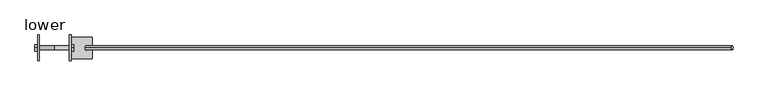
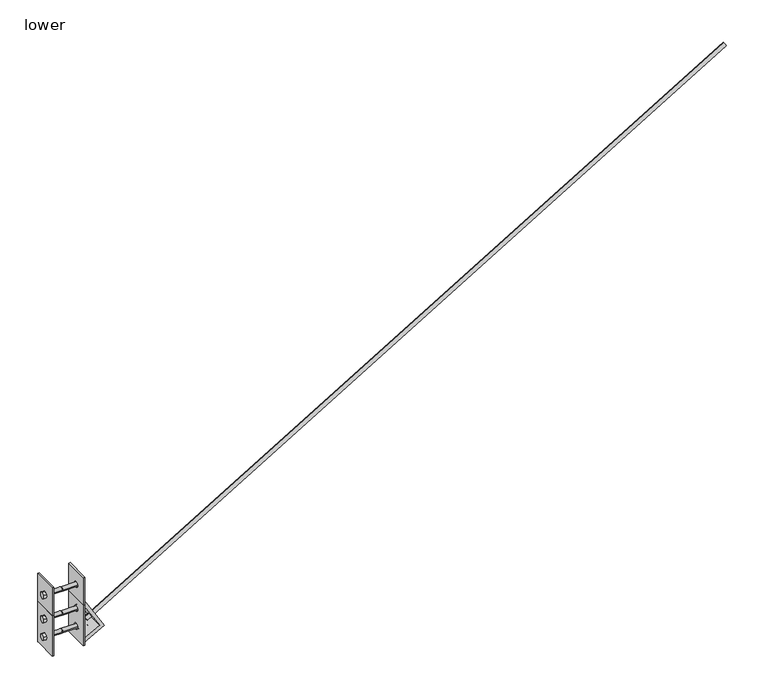
"""IFC4 building model written with IfcOpenShell, lengths in millimetres: fastener geometry, 060523 - W_P_C - Fastenings - Column Base & Top with X Bracing - Custom : lower."""

from ifc_helpers import new_model, si_unit, point, frame, frame_2d, origin, place, context, project, spatial, polyline, circle_curve, trimmed, segment, composite_curve, outline, extrude, source, transform, mapped, element, save
from ifc_brep_helpers import plane_surface, revolved_surface, advanced_brep


def lower_b6991e01(model_context):
    return source(origin(), model_context, "Body", "SolidModel", [
        extrude(outline(polyline([(-14.2875, 168.586392), (0.0, 176.8352839), (14.2875, 168.586392), (14.2875, 152.088608), (0.0, 143.8397161), (-14.2875, 152.088608), (-14.2875, 168.586392)])), frame((-90.4875, 0.0, 0.0), z_axis=(1.0, 0.0, 0.0), x_axis=(0.0, 1.0, 0.0)), (0.0, 0.0, 1.0), 12.7),
        extrude(outline(composite_curve([segment(trimmed(circle_curve(frame_2d((0.0, 160.3375)), 9.525), [point((-9.525, 160.3375))], [point((9.525, 160.3375))], False, "CARTESIAN"), True, "CONTINUOUS"), segment(trimmed(circle_curve(frame_2d((0.0, 160.3375)), 9.525), [point((9.525, 160.3375))], [point((-9.525, 160.3375))], False, "CARTESIAN"), True, "CONTINUOUS")], self_intersect=False)), frame((-77.7875, 0.0, 0.0), z_axis=(1.0, 0.0, 0.0), x_axis=(0.0, 1.0, 0.0)), (0.0, 0.0, 1.0), 76.2),
        extrude(outline(polyline([(-14.2875, 79.686392), (0.0, 87.9352839), (14.2875, 79.686392), (14.2875, 63.188608), (0.0, 54.9397161), (-14.2875, 63.188608), (-14.2875, 79.686392)])), frame((-90.4875, 0.0, 0.0), z_axis=(1.0, 0.0, 0.0), x_axis=(0.0, 1.0, 0.0)), (0.0, 0.0, 1.0), 12.7),
        extrude(outline(composite_curve([segment(trimmed(circle_curve(frame_2d((0.0, 71.4375)), 9.525), [point((-9.525, 71.4375))], [point((9.525, 71.4375))], False, "CARTESIAN"), True, "CONTINUOUS"), segment(trimmed(circle_curve(frame_2d((0.0, 71.4375)), 9.525), [point((9.525, 71.4375))], [point((-9.525, 71.4375))], False, "CARTESIAN"), True, "CONTINUOUS")], self_intersect=False)), frame((-77.7875, 0.0, 0.0), z_axis=(1.0, 0.0, 0.0), x_axis=(0.0, 1.0, 0.0)), (0.0, 0.0, 1.0), 76.2),
        extrude(outline(polyline([(-14.2875, 168.586392), (0.0, 176.8352839), (14.2875, 168.586392), (14.2875, 152.088608), (0.0, 143.8397161), (-14.2875, 152.088608), (-14.2875, 168.586392)])), frame((-90.4875, 0.0, 0.0), z_axis=(1.0, 0.0, 0.0), x_axis=(0.0, 1.0, 0.0)), (0.0, 0.0, 1.0), 12.7),
        extrude(outline(composite_curve([segment(trimmed(circle_curve(frame_2d((0.0, 160.3375)), 9.525), [point((-9.525, 160.3375))], [point((9.525, 160.3375))], False, "CARTESIAN"), True, "CONTINUOUS"), segment(trimmed(circle_curve(frame_2d((0.0, 160.3375)), 9.525), [point((9.525, 160.3375))], [point((-9.525, 160.3375))], False, "CARTESIAN"), True, "CONTINUOUS")], self_intersect=False)), frame((-77.7875, 0.0, 0.0), z_axis=(1.0, 0.0, 0.0), x_axis=(0.0, 1.0, 0.0)), (0.0, 0.0, 1.0), 76.2),
        advanced_brep(
        [(-77.7875, 60.325, 211.1375), (-77.7875, 60.325, 7.9375), (-77.7875, 52.3875, 7.9375), (-77.7875, -60.325, 7.9375), (-77.7875, -60.325, 211.1375), (-77.7875, 52.3875, 211.1375), (-77.7875, 13.890625, 160.3375), (-77.7875, -13.890625, 160.3375), (-77.7875, 13.890625, 71.4375), (-77.7875, -13.890625, 71.4375), (-69.85, -13.890625, 160.3375), (-69.85, 13.890625, 160.3375), (-69.85, 13.890625, 71.4375), (-69.85, -13.890625, 71.4375), (-69.85, 60.325, 211.1375), (-69.85, -60.325, 211.1375), (-69.85, -60.325, 7.9375), (-69.85, 60.325, 7.9375)],
        [
            (0, 1),
            (1, 2),
            (2, 3),
            (3, 4),
            (4, 5),
            (5, 0),
            (6, 7, circle_curve(frame((-77.7875, 0.0, 160.3375), z_axis=(1.0, 0.0, 0.0), x_axis=(0.0, 1.0, 0.0)), 13.890625)),
            (7, 6, circle_curve(frame((-77.7875, 0.0, 160.3375), z_axis=(1.0, 0.0, 0.0), x_axis=(0.0, 1.0, 0.0)), 13.890625)),
            (8, 9, circle_curve(frame((-77.7875, 0.0, 71.4375), z_axis=(1.0, 0.0, 0.0), x_axis=(0.0, 1.0, 0.0)), 13.890625)),
            (9, 8, circle_curve(frame((-77.7875, 0.0, 71.4375), z_axis=(1.0, 0.0, 0.0), x_axis=(0.0, 1.0, 0.0)), 13.890625)),
            (10, 11, circle_curve(frame((-69.85, 0.0, 160.3375), z_axis=(1.0, 0.0, 0.0), x_axis=(0.0, 1.0, 0.0)), 13.890625)),
            (11, 6),
            (7, 10),
            (11, 10, circle_curve(frame((-69.85, 0.0, 160.3375), z_axis=(1.0, 0.0, 0.0), x_axis=(0.0, 1.0, 0.0)), 13.890625)),
            (8, 12),
            (12, 13, circle_curve(frame((-69.85, 0.0, 71.4375), z_axis=(1.0, 0.0, 0.0), x_axis=(0.0, 1.0, 0.0)), 13.890625)),
            (13, 9),
            (13, 12, circle_curve(frame((-69.85, 0.0, 71.4375), z_axis=(1.0, 0.0, 0.0), x_axis=(0.0, 1.0, 0.0)), 13.890625)),
            (14, 15),
            (15, 16),
            (16, 17),
            (17, 14),
            (4, 15),
            (14, 0),
            (3, 16),
            (1, 17),
        ],
        [
            plane_surface(frame((-77.7875, -60.325, 211.1375), z_axis=(-1.0, 0.0, 0.0), x_axis=(0.0, -1.0, 0.0))),
            revolved_surface(polyline([(-77.7875, 13.890625, 160.3375), (-69.85, 13.890625, 160.3375)]), (-69.85, 0.0, 160.3375), (-1.0, 0.0, 0.0)),
            revolved_surface(polyline([(-77.7875, 13.890625, 71.4375), (-69.85, 13.890625, 71.4375)]), (-69.85, 0.0, 71.4375), (-1.0, 0.0, 0.0)),
            plane_surface(frame((-69.85, -60.325, 211.1375), z_axis=(1.0, 0.0, 0.0), x_axis=(0.0, 1.0, 0.0))),
            plane_surface(frame((-77.7875, 60.325, 211.1375), z_axis=(0.0, 0.0, 1.0), x_axis=(1.0, 0.0, 0.0))),
            plane_surface(frame((-77.7875, -60.325, 211.1375), z_axis=(0.0, -1.0, 0.0), x_axis=(1.0, 0.0, 0.0))),
            plane_surface(frame((-77.7875, -60.325, 7.9375), z_axis=(0.0, 0.0, -1.0), x_axis=(1.0, 0.0, 0.0))),
            plane_surface(frame((-77.7875, 60.325, 7.9375), z_axis=(0.0, 1.0, 0.0), x_axis=(1.0, 0.0, 0.0))),
        ],
        [
            (0, [[1, 2, 3, 4, 5, 6], [7, 8], [9, 10]]),
            (1, [[11, 12, -8, 13]]),
            (1, [[-7, -12, 14, -13]]),
            (2, [[-9, 15, 16, 17]]),
            (2, [[18, -15, -10, -17]]),
            (3, [[19, 20, 21, 22], [-14, -11], [-16, -18]]),
            (4, [[23, -19, 24, -6, -5]]),
            (5, [[25, -20, -23, -4]]),
            (6, [[26, -21, -25, -3, -2]]),
            (7, [[-24, -22, -26, -1]]),
        ],
    ),
        extrude(outline(polyline([(-14.2875, 168.586392), (0.0, 176.8352839), (14.2875, 168.586392), (14.2875, 152.088608), (0.0, 143.8397161), (-14.2875, 152.088608), (-14.2875, 168.586392)])), frame((77.7875, 0.0, 0.0), z_axis=(1.0, 0.0, 0.0), x_axis=(0.0, 1.0, 0.0)), (0.0, 0.0, 1.0), 12.7),
        extrude(outline(composite_curve([segment(trimmed(circle_curve(frame_2d((0.0, 160.3375)), 9.525), [point((-9.525, 160.3375))], [point((9.525, 160.3375))], False, "CARTESIAN"), True, "CONTINUOUS"), segment(trimmed(circle_curve(frame_2d((0.0, 160.3375)), 9.525), [point((9.525, 160.3375))], [point((-9.525, 160.3375))], False, "CARTESIAN"), True, "CONTINUOUS")], self_intersect=False)), frame((1.5875, 0.0, 0.0), z_axis=(1.0, 0.0, 0.0), x_axis=(0.0, 1.0, 0.0)), (0.0, 0.0, 1.0), 76.2),
        extrude(outline(polyline([(-14.2875, 79.686392), (0.0, 87.9352839), (14.2875, 79.686392), (14.2875, 63.188608), (0.0, 54.9397161), (-14.2875, 63.188608), (-14.2875, 79.686392)])), frame((77.7875, 0.0, 0.0), z_axis=(1.0, 0.0, 0.0), x_axis=(0.0, 1.0, 0.0)), (0.0, 0.0, 1.0), 12.7),
        extrude(outline(composite_curve([segment(trimmed(circle_curve(frame_2d((0.0, 71.4375)), 9.525), [point((-9.525, 71.4375))], [point((9.525, 71.4375))], False, "CARTESIAN"), True, "CONTINUOUS"), segment(trimmed(circle_curve(frame_2d((0.0, 71.4375)), 9.525), [point((9.525, 71.4375))], [point((-9.525, 71.4375))], False, "CARTESIAN"), True, "CONTINUOUS")], self_intersect=False)), frame((1.5875, 0.0, 0.0), z_axis=(1.0, 0.0, 0.0), x_axis=(0.0, 1.0, 0.0)), (0.0, 0.0, 1.0), 76.2),
        extrude(outline(polyline([(-14.2875, 168.586392), (0.0, 176.8352839), (14.2875, 168.586392), (14.2875, 152.088608), (0.0, 143.8397161), (-14.2875, 152.088608), (-14.2875, 168.586392)])), frame((77.7875, 0.0, 0.0), z_axis=(1.0, 0.0, 0.0), x_axis=(0.0, 1.0, 0.0)), (0.0, 0.0, 1.0), 12.7),
        extrude(outline(composite_curve([segment(trimmed(circle_curve(frame_2d((0.0, 160.3375)), 9.525), [point((-9.525, 160.3375))], [point((9.525, 160.3375))], False, "CARTESIAN"), True, "CONTINUOUS"), segment(trimmed(circle_curve(frame_2d((0.0, 160.3375)), 9.525), [point((9.525, 160.3375))], [point((-9.525, 160.3375))], False, "CARTESIAN"), True, "CONTINUOUS")], self_intersect=False)), frame((1.5875, 0.0, 0.0), z_axis=(1.0, 0.0, 0.0), x_axis=(0.0, 1.0, 0.0)), (0.0, 0.0, 1.0), 76.2),
        advanced_brep(
        [(77.7875, 60.325, 211.1375), (77.7875, 52.3875, 211.1375), (77.7875, -60.325, 211.1375), (77.7875, -60.325, 7.9375), (77.7875, 52.3875, 7.9375), (77.7875, 60.325, 7.9375), (77.7875, 13.890625, 71.4375), (77.7875, -13.890625, 71.4375), (77.7875, 13.890625, 160.3375), (77.7875, -13.890625, 160.3375), (69.85, -13.890625, 160.3375), (69.85, 13.890625, 160.3375), (69.85, -13.890625, 71.4375), (69.85, 13.890625, 71.4375), (69.85, 60.325, 211.1375), (69.85, 60.325, 7.9375), (69.85, -60.325, 7.9375), (69.85, -60.325, 211.1375)],
        [
            (0, 1),
            (1, 2),
            (2, 3),
            (3, 4),
            (4, 5),
            (5, 0),
            (6, 7, circle_curve(frame((77.7875, 0.0, 71.4375), z_axis=(-1.0, 0.0, 0.0), x_axis=(0.0, 1.0, 0.0)), 13.890625)),
            (7, 6, circle_curve(frame((77.7875, 0.0, 71.4375), z_axis=(-1.0, 0.0, 0.0), x_axis=(0.0, 1.0, 0.0)), 13.890625)),
            (8, 9, circle_curve(frame((77.7875, 0.0, 160.3375), z_axis=(-1.0, 0.0, 0.0), x_axis=(0.0, 1.0, 0.0)), 13.890625)),
            (9, 8, circle_curve(frame((77.7875, 0.0, 160.3375), z_axis=(-1.0, 0.0, 0.0), x_axis=(0.0, 1.0, 0.0)), 13.890625)),
            (10, 9),
            (8, 11),
            (11, 10, circle_curve(frame((69.85, 0.0, 160.3375), z_axis=(-1.0, 0.0, 0.0), x_axis=(0.0, 1.0, 0.0)), 13.890625)),
            (10, 11, circle_curve(frame((69.85, 0.0, 160.3375), z_axis=(-1.0, 0.0, 0.0), x_axis=(0.0, 1.0, 0.0)), 13.890625)),
            (7, 12),
            (12, 13, circle_curve(frame((69.85, 0.0, 71.4375), z_axis=(-1.0, 0.0, 0.0), x_axis=(0.0, 1.0, 0.0)), 13.890625)),
            (13, 6),
            (13, 12, circle_curve(frame((69.85, 0.0, 71.4375), z_axis=(-1.0, 0.0, 0.0), x_axis=(0.0, 1.0, 0.0)), 13.890625)),
            (14, 15),
            (15, 16),
            (16, 17),
            (17, 14),
            (0, 14),
            (17, 2),
            (16, 3),
            (15, 5),
        ],
        [
            plane_surface(frame((77.7875, -60.325, 211.1375), z_axis=(1.0, 0.0, 0.0), x_axis=(0.0, -1.0, 0.0))),
            revolved_surface(polyline([(77.7875, 13.890625, 160.3375), (69.85, 13.890625, 160.3375)]), (69.85, 0.0, 160.3375), (1.0, 0.0, 0.0)),
            revolved_surface(polyline([(77.7875, 13.890625, 71.4375), (69.85, 13.890625, 71.4375)]), (69.85, 0.0, 71.4375), (1.0, 0.0, 0.0)),
            plane_surface(frame((69.85, -60.325, 211.1375), z_axis=(-1.0, 0.0, 0.0), x_axis=(0.0, 1.0, 0.0))),
            plane_surface(frame((77.7875, 60.325, 211.1375), z_axis=(0.0, 0.0, 1.0), x_axis=(-1.0, 0.0, 0.0))),
            plane_surface(frame((77.7875, -60.325, 211.1375), z_axis=(0.0, -1.0, 0.0), x_axis=(-1.0, 0.0, 0.0))),
            plane_surface(frame((77.7875, -60.325, 7.9375), z_axis=(0.0, 0.0, -1.0), x_axis=(-1.0, 0.0, 0.0))),
            plane_surface(frame((77.7875, 60.325, 7.9375), z_axis=(0.0, 1.0, 0.0), x_axis=(-1.0, 0.0, 0.0))),
        ],
        [
            (0, [[1, 2, 3, 4, 5, 6], [7, 8], [9, 10]]),
            (1, [[11, -9, 12, 13]]),
            (1, [[-11, 14, -12, -10]]),
            (2, [[15, 16, 17, -8]]),
            (2, [[-15, -7, -17, 18]]),
            (3, [[19, 20, 21, 22], [-18, -16], [-13, -14]]),
            (4, [[-2, -1, 23, -22, 24]]),
            (5, [[-3, -24, -21, 25]]),
            (6, [[-5, -4, -25, -20, 26]]),
            (7, [[-6, -26, -19, -23]]),
        ],
    ),
        extrude(outline(polyline([(-14.2875, 289.236392), (0.0, 297.4852839), (14.2875, 289.236392), (14.2875, 272.738608), (0.0, 264.4897161), (-14.2875, 272.738608), (-14.2875, 289.236392)])), frame((-90.4875, 0.0, 0.0), z_axis=(1.0, 0.0, 0.0), x_axis=(0.0, 1.0, 0.0)), (0.0, 0.0, 1.0), 12.7),
        extrude(outline(composite_curve([segment(trimmed(circle_curve(frame_2d((0.0, 280.9875)), 9.525), [point((-9.525, 280.9875))], [point((9.525, 280.9875))], False, "CARTESIAN"), True, "CONTINUOUS"), segment(trimmed(circle_curve(frame_2d((0.0, 280.9875)), 9.525), [point((9.525, 280.9875))], [point((-9.525, 280.9875))], False, "CARTESIAN"), True, "CONTINUOUS")], self_intersect=False)), frame((-77.7875, 0.0, 0.0), z_axis=(1.0, 0.0, 0.0), x_axis=(0.0, 1.0, 0.0)), (0.0, 0.0, 1.0), 76.2),
        advanced_brep(
        [(-77.7875, 60.325, 350.8375), (-77.7875, 60.325, 211.1375), (-77.7875, -52.3875, 211.1375), (-77.7875, -60.325, 211.1375), (-77.7875, -60.325, 350.8375), (-77.7875, -52.3875, 350.8375), (-77.7875, 13.890625, 280.9875), (-77.7875, -13.890625, 280.9875), (-69.85, 60.325, 350.8375), (-69.85, -60.325, 350.8375), (-69.85, -60.325, 211.1375), (-69.85, 60.325, 211.1375), (-69.85, -13.890625, 280.9875), (-69.85, 13.890625, 280.9875)],
        [
            (0, 1),
            (1, 2),
            (2, 3),
            (3, 4),
            (4, 5),
            (5, 0),
            (6, 7, circle_curve(frame((-77.7875, 0.0, 280.9875), z_axis=(1.0, 0.0, 0.0), x_axis=(0.0, 1.0, 0.0)), 13.890625)),
            (7, 6, circle_curve(frame((-77.7875, 0.0, 280.9875), z_axis=(1.0, 0.0, 0.0), x_axis=(0.0, 1.0, 0.0)), 13.890625)),
            (8, 9),
            (9, 10),
            (10, 11),
            (11, 8),
            (12, 13, circle_curve(frame((-69.85, 0.0, 280.9875), z_axis=(-1.0, 0.0, 0.0), x_axis=(0.0, 1.0, 0.0)), 13.890625)),
            (13, 12, circle_curve(frame((-69.85, 0.0, 280.9875), z_axis=(-1.0, 0.0, 0.0), x_axis=(0.0, 1.0, 0.0)), 13.890625)),
            (4, 9),
            (8, 0),
            (3, 10),
            (1, 11),
            (13, 6),
            (7, 12),
        ],
        [
            plane_surface(frame((-77.7875, -60.325, 350.8375), z_axis=(-1.0, 0.0, 0.0), x_axis=(0.0, -1.0, 0.0))),
            plane_surface(frame((-69.85, -60.325, 350.8375), z_axis=(1.0, 0.0, 0.0), x_axis=(0.0, 1.0, 0.0))),
            plane_surface(frame((-77.7875, 60.325, 350.8375), z_axis=(0.0, 0.0, 1.0), x_axis=(1.0, 0.0, 0.0))),
            plane_surface(frame((-77.7875, -60.325, 350.8375), z_axis=(0.0, -1.0, 0.0), x_axis=(1.0, 0.0, 0.0))),
            plane_surface(frame((-77.7875, -60.325, 211.1375), z_axis=(0.0, 0.0, -1.0), x_axis=(1.0, 0.0, 0.0))),
            plane_surface(frame((-77.7875, 60.325, 211.1375), z_axis=(0.0, 1.0, 0.0), x_axis=(1.0, 0.0, 0.0))),
            revolved_surface(polyline([(-77.7875, 13.890625, 280.9875), (-69.85, 13.890625, 280.9875)]), (-69.85, 0.0, 280.9875), (-1.0, 0.0, 0.0)),
        ],
        [
            (0, [[1, 2, 3, 4, 5, 6], [7, 8]]),
            (1, [[9, 10, 11, 12], [13, 14]]),
            (2, [[15, -9, 16, -6, -5]]),
            (3, [[17, -10, -15, -4]]),
            (4, [[18, -11, -17, -3, -2]]),
            (5, [[-16, -12, -18, -1]]),
            (6, [[-14, 19, -8, 20]]),
            (6, [[-7, -19, -13, -20]]),
        ],
    ),
        extrude(outline(polyline([(-14.2875, 289.236392), (0.0, 297.4852839), (14.2875, 289.236392), (14.2875, 272.738608), (0.0, 264.4897161), (-14.2875, 272.738608), (-14.2875, 289.236392)])), frame((77.7875, 0.0, 0.0), z_axis=(1.0, 0.0, 0.0), x_axis=(0.0, 1.0, 0.0)), (0.0, 0.0, 1.0), 12.7),
        extrude(outline(composite_curve([segment(trimmed(circle_curve(frame_2d((0.0, 280.9875)), 9.525), [point((-9.525, 280.9875))], [point((9.525, 280.9875))], False, "CARTESIAN"), True, "CONTINUOUS"), segment(trimmed(circle_curve(frame_2d((0.0, 280.9875)), 9.525), [point((9.525, 280.9875))], [point((-9.525, 280.9875))], False, "CARTESIAN"), True, "CONTINUOUS")], self_intersect=False)), frame((1.5875, 0.0, 0.0), z_axis=(1.0, 0.0, 0.0), x_axis=(0.0, 1.0, 0.0)), (0.0, 0.0, 1.0), 76.2),
        advanced_brep(
        [(77.7875, 60.325, 350.8375), (77.7875, -52.3875, 350.8375), (77.7875, -60.325, 350.8375), (77.7875, -60.325, 211.1375), (77.7875, -52.3875, 211.1375), (77.7875, 60.325, 211.1375), (77.7875, 13.890625, 280.9875), (77.7875, -13.890625, 280.9875), (69.85, 60.325, 350.8375), (69.85, 60.325, 211.1375), (69.85, -60.325, 211.1375), (69.85, -60.325, 350.8375), (69.85, -13.890625, 280.9875), (69.85, 13.890625, 280.9875)],
        [
            (0, 1),
            (1, 2),
            (2, 3),
            (3, 4),
            (4, 5),
            (5, 0),
            (6, 7, circle_curve(frame((77.7875, 0.0, 280.9875), z_axis=(-1.0, 0.0, 0.0), x_axis=(0.0, 1.0, 0.0)), 13.890625)),
            (7, 6, circle_curve(frame((77.7875, 0.0, 280.9875), z_axis=(-1.0, 0.0, 0.0), x_axis=(0.0, 1.0, 0.0)), 13.890625)),
            (8, 9),
            (9, 10),
            (10, 11),
            (11, 8),
            (12, 13, circle_curve(frame((69.85, 0.0, 280.9875), z_axis=(1.0, 0.0, 0.0), x_axis=(0.0, 1.0, 0.0)), 13.890625)),
            (13, 12, circle_curve(frame((69.85, 0.0, 280.9875), z_axis=(1.0, 0.0, 0.0), x_axis=(0.0, 1.0, 0.0)), 13.890625)),
            (0, 8),
            (11, 2),
            (10, 3),
            (9, 5),
            (12, 7),
            (6, 13),
        ],
        [
            plane_surface(frame((77.7875, -60.325, 350.8375), z_axis=(1.0, 0.0, 0.0), x_axis=(0.0, -1.0, 0.0))),
            plane_surface(frame((69.85, -60.325, 350.8375), z_axis=(-1.0, 0.0, 0.0), x_axis=(0.0, 1.0, 0.0))),
            plane_surface(frame((77.7875, 60.325, 350.8375), z_axis=(0.0, 0.0, 1.0), x_axis=(-1.0, 0.0, 0.0))),
            plane_surface(frame((77.7875, -60.325, 350.8375), z_axis=(0.0, -1.0, 0.0), x_axis=(-1.0, 0.0, 0.0))),
            plane_surface(frame((77.7875, -60.325, 211.1375), z_axis=(0.0, 0.0, -1.0), x_axis=(-1.0, 0.0, 0.0))),
            plane_surface(frame((77.7875, 60.325, 211.1375), z_axis=(0.0, 1.0, 0.0), x_axis=(-1.0, 0.0, 0.0))),
            revolved_surface(polyline([(77.7875, 13.890625, 280.9875), (69.85, 13.890625, 280.9875)]), (69.85, 0.0, 280.9875), (1.0, 0.0, 0.0)),
        ],
        [
            (0, [[1, 2, 3, 4, 5, 6], [7, 8]]),
            (1, [[9, 10, 11, 12], [13, 14]]),
            (2, [[-2, -1, 15, -12, 16]]),
            (3, [[-3, -16, -11, 17]]),
            (4, [[-5, -4, -17, -10, 18]]),
            (5, [[-6, -18, -9, -15]]),
            (6, [[19, -7, 20, -13]]),
            (6, [[-19, -14, -20, -8]]),
        ],
    ),
        extrude(outline(composite_curve([segment(trimmed(circle_curve(frame_2d((0.0, -9.525)), 9.525), [point((0.0, -19.05))], [point((0.0, 0.0))], False, "CARTESIAN"), True, "CONTINUOUS"), segment(trimmed(circle_curve(frame_2d((0.0, -9.525)), 9.525), [point((0.0, 0.0))], [point((0.0, -19.05))], False, "CARTESIAN"), True, "CONTINUOUS")], self_intersect=False)), frame((121.5297809, 0.0, 84.6558969), z_axis=(0.8571673007021132, 0.0, 0.5150380749100526), x_axis=(0.0, -1.0, 0.0)), (0.0, 0.0, 1.0), 3543.3),
        advanced_brep(
        [(175.4460516, -50.8, 68.8992672), (77.7875, -50.8, 231.430391), (77.7875, -50.8, 200.6074271), (153.29752, -50.8, 74.93765), (77.7875, -50.8, 33.9390543), (77.7875, -50.8, 15.875), (175.4460516, 50.8, 68.8992672), (77.7875, 50.8, 15.875), (77.7875, 50.8, 33.9390543), (153.29752, 50.8, 74.93765), (77.7875, 50.8, 200.6074271), (77.7875, 50.8, 231.430391), (154.8010723, 0.0, 103.2582828), (143.7631626, 0.0, 121.6284495), (130.1556317, 0.0, 113.45222), (141.1935414, 0.0, 95.0820533), (123.5760275, 0.0, 58.8001963), (122.8784665, 0.0, 58.4214515), (130.4533618, 0.0, 44.4702298), (131.1509229, 0.0, 44.8489746)],
        [
            (0, 1),
            (1, 2),
            (2, 3),
            (3, 4),
            (4, 5),
            (5, 0),
            (6, 7),
            (7, 8),
            (8, 9),
            (9, 10),
            (10, 11),
            (11, 6),
            (0, 6),
            (11, 1),
            (12, 13, circle_curve(frame((149.2821174, 0.0, 112.4433661), z_axis=(-0.8571673007021132, 0.0, -0.5150380749100526), x_axis=(-0.5150380749100526, 0.0, 0.8571673007021132)), 10.715625)),
            (13, 12, circle_curve(frame((149.2821174, 0.0, 112.4433661), z_axis=(-0.8571673007021132, 0.0, -0.5150380749100526), x_axis=(-0.5150380749100526, 0.0, 0.8571673007021132)), 10.715625)),
            (10, 2),
            (9, 3),
            (14, 15, circle_curve(frame((135.6745865, 0.0, 104.2671367), z_axis=(0.8571673007021132, 0.0, 0.5150380749100526), x_axis=(-0.5150380749100526, 0.0, 0.8571673007021132)), 10.715625)),
            (15, 14, circle_curve(frame((135.6745865, 0.0, 104.2671367), z_axis=(0.8571673007021132, 0.0, 0.5150380749100526), x_axis=(-0.5150380749100526, 0.0, 0.8571673007021132)), 10.715625)),
            (8, 4),
            (16, 17, circle_curve(frame((123.227247, 0.0, 58.6108239), z_axis=(0.47715876025960574, 0.0, -0.8788171126619669), x_axis=(0.8788171126619669, 0.0, 0.47715876025960574)), 0.396875)),
            (17, 16, circle_curve(frame((123.227247, 0.0, 58.6108239), z_axis=(0.47715876025960574, 0.0, -0.8788171126619669), x_axis=(0.8788171126619669, 0.0, 0.47715876025960574)), 0.396875)),
            (7, 5),
            (18, 19, circle_curve(frame((130.8021423, 0.0, 44.6596022), z_axis=(-0.47715876025960574, 0.0, 0.8788171126619669), x_axis=(0.8788171126619669, 0.0, 0.47715876025960574)), 0.396875)),
            (19, 18, circle_curve(frame((130.8021423, 0.0, 44.6596022), z_axis=(-0.47715876025960574, 0.0, 0.8788171126619669), x_axis=(0.8788171126619669, 0.0, 0.47715876025960574)), 0.396875)),
            (12, 15),
            (14, 13),
            (18, 17),
            (16, 19),
        ],
        [
            plane_surface(frame((77.7875, -50.8, 231.430391), z_axis=(0.0, -1.0, 0.0), x_axis=(-0.5150380749100526, 0.0, 0.8571673007021132))),
            plane_surface(frame((77.7875, 50.8, 231.430391), z_axis=(0.0, 1.0, 0.0), x_axis=(0.5150380749100526, 0.0, -0.8571673007021132))),
            plane_surface(frame((175.4460516, -50.8, 68.8992672), z_axis=(0.8571673007021132, 0.0, 0.5150380749100526), x_axis=(0.0, 1.0, 0.0))),
            plane_surface(frame((77.7875, -50.8, 231.430391), z_axis=(-1.0, 0.0, 0.0), x_axis=(0.0, 1.0, 0.0))),
            plane_surface(frame((77.7875, -50.8, 200.6074271), z_axis=(-0.8571673007021139, 0.0, -0.5150380749100517), x_axis=(0.0, 1.0, 0.0))),
            plane_surface(frame((153.29752, -50.8, 74.93765), z_axis=(-0.47715876025960563, 0.0, 0.8788171126619669), x_axis=(0.0, 1.0, 0.0))),
            plane_surface(frame((77.7875, -50.8, 33.9390543), z_axis=(-1.0, 0.0, 0.0), x_axis=(0.0, 1.0, 0.0))),
            plane_surface(frame((77.7875, -50.8, 15.875), z_axis=(0.477158760259606, 0.0, -0.8788171126619667), x_axis=(0.0, 1.0, 0.0))),
            revolved_surface(polyline([(130.15563164620562, 0.0, 113.45222002718884), (143.76316260021085, 0.0, 121.62844949964908)]), (149.2821174, 0.0, 112.4433661), (-0.8571673007021132, 0.0, -0.5150380749100526)),
            revolved_surface(polyline([(123.57602749491133, 0.0, 58.80019629723708), (131.15092285819438, 0.0, 44.848974552392434)]), (130.8021423, 0.0, 44.6596022), (-0.47715876025960574, 0.0, 0.8788171126619669)),
        ],
        [
            (0, [[1, 2, 3, 4, 5, 6]]),
            (1, [[7, 8, 9, 10, 11, 12]]),
            (2, [[-1, 13, -12, 14], [15, 16]]),
            (3, [[-2, -14, -11, 17]]),
            (4, [[-3, -17, -10, 18], [19, 20]]),
            (5, [[-4, -18, -9, 21], [22, 23]]),
            (6, [[-5, -21, -8, 24]]),
            (7, [[-6, -24, -7, -13], [25, 26]]),
            (8, [[27, -19, 28, -15]]),
            (8, [[-27, -16, -28, -20]]),
            (9, [[29, -22, 30, -25]]),
            (9, [[-29, -26, -30, -23]]),
        ],
    ),
    ])


if __name__ == "__main__":
    model = new_model("IFC4")
    model_context = context("Model", 3, world=origin())
    ifc_project = project(units=[si_unit("LENGTHUNIT", "METRE", prefix="MILLI")], contexts=[model_context])
    site = spatial("IfcSite", under=ifc_project)
    building = spatial("IfcBuilding", under=site)
    placement = place(None, origin())
    lower_shape = lower_b6991e01(model_context)
    element("IfcFastener", 1, ObjectType="060523 - W_P_C - Fastenings - Column Base & Top with X Bracing - Custom : lower", at=placement, inside=building, context=model_context, shape_type="MappedRepresentation", body=[
        mapped(lower_shape, transform((0.0, 0.0, 0.0), x_axis=(1.0, 0.0, 0.0), y_axis=(0.0, 1.0, 0.0), z_axis=(0.0, 0.0, 1.0))),
    ])
    save(model, "model.ifc")

# Revit data of these elements
# Type "060523 - W_P_C - Fastenings - Column Base & Top with X Bracing - Custom : lower"
#   Width - Top = 0' - 5 1/2"
#   Top/Bottom Plate Thickness = 0' - 0 5/16"
#   Top/Bottom Plate - Width = 0' - 7 1/2"
#   Rod Radius = 0' - 0 3/8"
#   Rod Length [instance default] = 11' - 4"
#   Plate Thickness = 0' - 0 5/16"
#   Offset - Upper Plate 2 = 0' - 0"
#   Height of Plate = 0' - 8"
#   Width - Bottom = 0' - 5 1/2"
#   Plate Width = 0' - 4 3/4"
#   Bracket Width = 0' - 4"
#   Bracket Thickness = 0' - 0 5/8"
#   Bracket Offset in X = 0' - 3 1/16"
#   Bracket Offset in Y = 0' - 0 3/8"
#   Bracket Offset = 0' - 0 5/8"
#   Bracket Leg = 0' - 4 3/8"
#   Bracket Hole Radius - Up = 0' - 0 27/64"
#   Bracket Hole Radius - Down = 0' - 0 1/64"
#   Bracket Hole Offset = 0' - 2"
#   Beam Width = 0' - 7 3/8"
#   Angle 2 = 31.00°
#   Angle 1 = 118.50°
#   Top Plate Visible = no
#   Rod Visibility = yes
#   Plate Visibility - Upper Right 2 = no
#   Plate Visibility - Upper Right 1 = yes
#   Plate Visibility - Upper Left 2 = no
#   Plate Visibility - Upper Left 1 = yes
#   Plate Visibility - Lower Right 2 = no
#   Plate Visibility - Lower Right 1 = yes
#   Plate Visibility - Lower Left 2 = no
#   Plate Visibility - Lower Left 1 = yes
#   Bracket Visibility = yes
#   Bottom Plate Visible = no
#   Upper Plates - 2 = element 1925091
#   Upper Plates - 1 = element 1925091
#   Rod Material = X-BRACING: 3/4" DIA. THREADED STEEL ROD (RAW) W/ TURNBUCKLE (NUTS AT STEEL ANGLE)
#   Lower Plates = element 1925092
#   Bracket Material = 5/8" STEEL ANGLE (RAW STEEL)
#   URL = ""
# Element 1 (IfcFastener, "060523 - W_P_C - Fastenings - Column Base & Top with X Bracing - Custom : lower")
#   Rod Length = 11' - 6"
#   Materials on its faces: "3/4\" LAG BOLT (THRU BOLT IF PLATE ON OPP. SIDE OF STRUCT MEMBER)", "5/16\" STEEL PLATE (RAW STEEL)", "5/8\" STEEL ANGLE (RAW STEEL)", "X-BRACING: 3/4\" DIA. THREADED STEEL ROD (RAW) W/ TURNBUCKLE (NUTS AT STEEL ANGLE)"
# Materials
#   "X-BRACING: 3/4\" DIA. THREADED STEEL ROD (RAW) W/ TURNBUCKLE (NUTS AT STEEL ANGLE)": class "Generic", colour RGB 212 212 212, transparency 0, Cost = 0
#   "5/8\" STEEL ANGLE (RAW STEEL)": class "Generic", colour RGB 195 195 195, transparency 0, Cost = 0
#   "3/4\" LAG BOLT (THRU BOLT IF PLATE ON OPP. SIDE OF STRUCT MEMBER)": class "Generic", colour RGB 120 120 120, transparency 0, Cost = 0
#   "5/16\" STEEL PLATE (RAW STEEL)": class "Generic", colour RGB 232 232 232, transparency 0, Cost = 0
